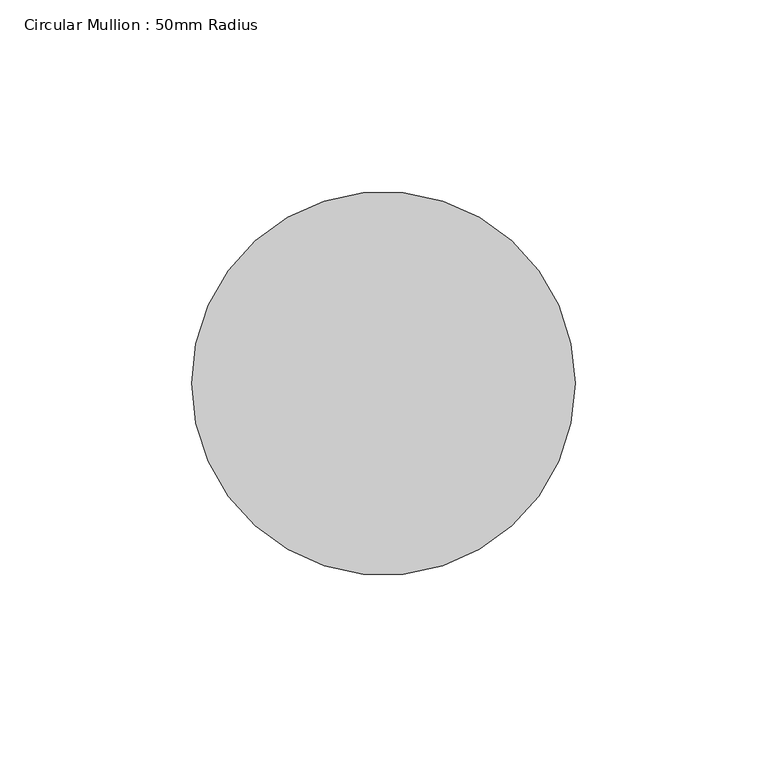
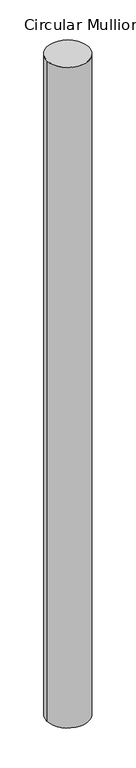
"""IFC4 building model written with IfcOpenShell, lengths in millimetres: member geometry, Circular Mullion : 50mm Radius."""

from ifc_helpers import new_model, si_unit, point, frame, origin, origin_2d, place, context, project, spatial, circle_curve, trimmed, segment, composite_curve, outline, extrude, source, transform, mapped, element, save


def circular_mullion_50mm_radius_82eff083(model_context):
    return source(origin(), model_context, "Body", "SweptSolid", [
        extrude(outline(composite_curve([segment(trimmed(circle_curve(origin_2d(), 50.0), [point((50.0, 0.0))], [point((-50.0, 0.0))], False, "CARTESIAN"), True, "CONTINUOUS"), segment(trimmed(circle_curve(origin_2d(), 50.0), [point((-50.0, 0.0))], [point((50.0, 0.0))], False, "CARTESIAN"), True, "CONTINUOUS")], self_intersect=False)), frame((0.0, 0.0, -1673.9080104), z_axis=(0.0, 0.0, 1.0), x_axis=(1.0, 0.0, 0.0)), (0.0, 0.0, 1.0), 1673.9080104),
    ])


if __name__ == "__main__":
    model = new_model("IFC4")
    model_context = context("Model", 3, world=origin())
    ifc_project = project(units=[si_unit("LENGTHUNIT", "METRE", prefix="MILLI")], contexts=[model_context])
    site = spatial("IfcSite", under=ifc_project)
    building = spatial("IfcBuilding", under=site)
    placement = place(None, origin())
    circular_mullion_50mm_radius_shape = circular_mullion_50mm_radius_82eff083(model_context)
    element("IfcMember", 1, ObjectType="Circular Mullion : 50mm Radius", at=placement, inside=building, context=model_context, shape_type="MappedRepresentation", body=[
        mapped(circular_mullion_50mm_radius_shape, transform((0.0, 0.0, 0.0), x_axis=(1.0, 0.0, 0.0), y_axis=(0.0, 1.0, 0.0), z_axis=(0.0, 0.0, 1.0))),
    ])
    save(model, "model.ifc")

# Revit data of these elements
# Type "Circular Mullion : 50mm Radius"
#   built-in parameter 1007350 = 0.164042 (stored number, unit not read)
# Element 1 (IfcMember, "Circular Mullion : 50mm Radius")
#   Materials on its faces: "Aluminium"
# Materials
#   "Aluminium": class "Metal", colour RGB 247 247 247, transparency 0, Description = "Aluminium 6061", Cost = 0
